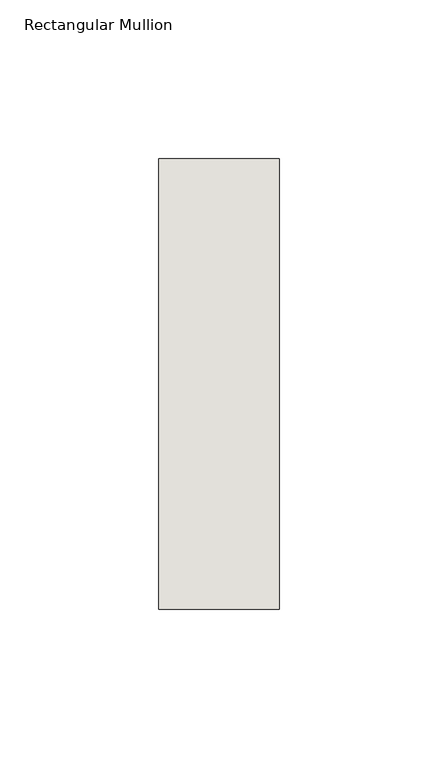
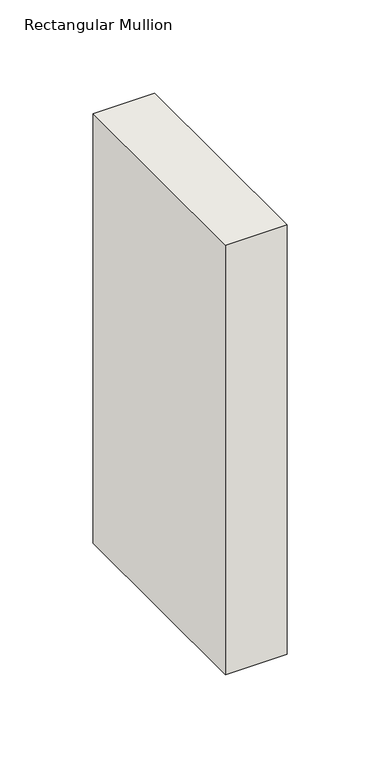
"""IFC4 building model written with IfcOpenShell, lengths in millimetres: wall geometry, Rectangular Mullion : NLRS_21_CWM_hsb-regel 38x142_gen_rsf."""

from ifc_helpers import new_model, si_unit, frame, origin, place, context, project, spatial, polyline, outline, extrude, source, transform, mapped, element, save


def rectangular_mullion_8622cd22(model_context):
    return source(origin(), model_context, "Body", "SweptSolid", [
        extrude(outline(polyline([(0.0, -71.0), (-38.0, -71.0), (-38.0, 71.0), (0.0, 71.0), (0.0, -71.0)])), frame((0.0, 0.0, -280.9999997), z_axis=(0.0, 0.0, 1.0), x_axis=(1.0, 0.0, 0.0)), (0.0, 0.0, 1.0), 280.9999997),
    ])


if __name__ == "__main__":
    model = new_model("IFC4")
    model_context = context("Model", 3, world=origin())
    ifc_project = project(units=[si_unit("LENGTHUNIT", "METRE", prefix="MILLI")], contexts=[model_context])
    site = spatial("IfcSite", under=ifc_project)
    building = spatial("IfcBuilding", under=site)
    placement = place(None, origin())
    rectangular_mullion_shape = rectangular_mullion_8622cd22(model_context)
    element("IfcWall", 1, ObjectType="Rectangular Mullion : NLRS_21_CWM_hsb-regel 38x142_gen_rsf", at=placement, inside=building, context=model_context, shape_type="MappedRepresentation", body=[
        mapped(rectangular_mullion_shape, transform((0.0, 0.0, 0.0), x_axis=(1.0, 0.0, 0.0), y_axis=(0.0, 1.0, 0.0), z_axis=(0.0, 0.0, 1.0))),
    ])
    save(model, "model.ifc")

# Revit data of these elements
# Type "Rectangular Mullion : NLRS_21_CWM_hsb-regel 38x142_gen_rsf"
#   Type IfcGUID = "07M7mRoiH1CR8m_RSKIwpF"
#   Assembly Code = "21.10"
#   IfcExportAs = "IfcWall"
#   built-in parameter 1007322 = 0.465879 (stored number, unit not read)
#   built-in parameter 1007321 = 0.062336 (stored number, unit not read)
#   built-in parameter 1007320 = 0.062336 (stored number, unit not read)
# Element 1 (IfcWall, "Rectangular Mullion : NLRS_21_CWM_hsb-regel 38x142_gen_rsf")
#   Materials on its faces: "NLRS_i2_hout naaldhout vuren_gen_rsf"
# Materials
#   "NLRS_i2_hout naaldhout vuren_gen_rsf": class "I - Hout", colour RGB 234 199 147, transparency 0, Keynote = "i2", Manufacturer = "Revit Standards Foundation", URL = "www.revitstandards.org", Description = "hout vuren", Cost = 0
